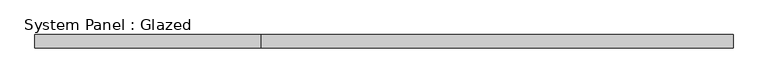
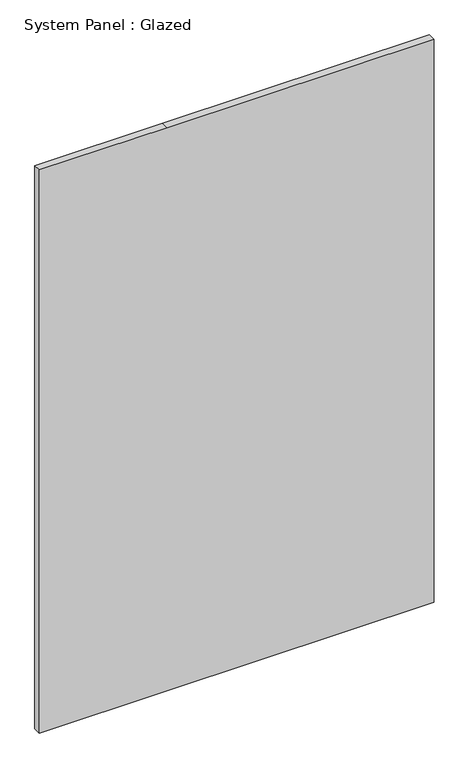
"""IFC4 building model written with IfcOpenShell, lengths in millimetres: plate geometry, System Panel : Glazed."""

from ifc_helpers import new_model, si_unit, frame, origin, place, context, project, spatial, polyline, outline, extrude, source, transform, mapped, element, save


def system_panel_glazed_0009e1a4(model_context):
    return source(origin(), model_context, "Body", "SweptSolid", [
        extrude(outline(polyline([(0.0, -676.275), (0.0, -238.125), (0.0, 676.275), (2038.35, 676.275), (2038.35, -238.125), (2038.35, -676.275), (0.0, -676.275)])), frame((0.0, -44.45, 0.0), z_axis=(0.0, 1.0, 0.0), x_axis=(0.0, 0.0, 1.0)), (0.0, 0.0, 1.0), 25.4),
    ])


if __name__ == "__main__":
    model = new_model("IFC4")
    model_context = context("Model", 3, world=origin())
    ifc_project = project(units=[si_unit("LENGTHUNIT", "METRE", prefix="MILLI")], contexts=[model_context])
    site = spatial("IfcSite", under=ifc_project)
    building = spatial("IfcBuilding", under=site)
    placement = place(None, origin())
    system_panel_glazed_shape = system_panel_glazed_0009e1a4(model_context)
    element("IfcPlate", 1, ObjectType="System Panel : Glazed", at=placement, inside=building, context=model_context, shape_type="MappedRepresentation", body=[
        mapped(system_panel_glazed_shape, transform((0.0, 0.0, 0.0), x_axis=(1.0, 0.0, 0.0), y_axis=(0.0, 1.0, 0.0), z_axis=(0.0, 0.0, 1.0))),
    ])
    save(model, "model.ifc")

# Revit data of these elements
# Type "System Panel : Glazed"
#   Construction Type Id = "GSP4R"
#   Analytic Construction = "1/8 in Pilkington single glazing"
#   Visual Light Transmittance = 0.9
#   Solar Heat Gain Coefficient = 0.86
#   Heat Transfer Coefficient (U) = 1.18115 BTU/(h·ft²·°F)
#   Define Thermal Properties by = 1
# Element 1 (IfcPlate, "System Panel : Glazed")
#   Materials on its faces: "Glass"
# Materials
#   "Glass": class "Glass", colour RGB 0 0 255, transparency 0.75, Description = "Soda Lime Glass", Cost = 0
